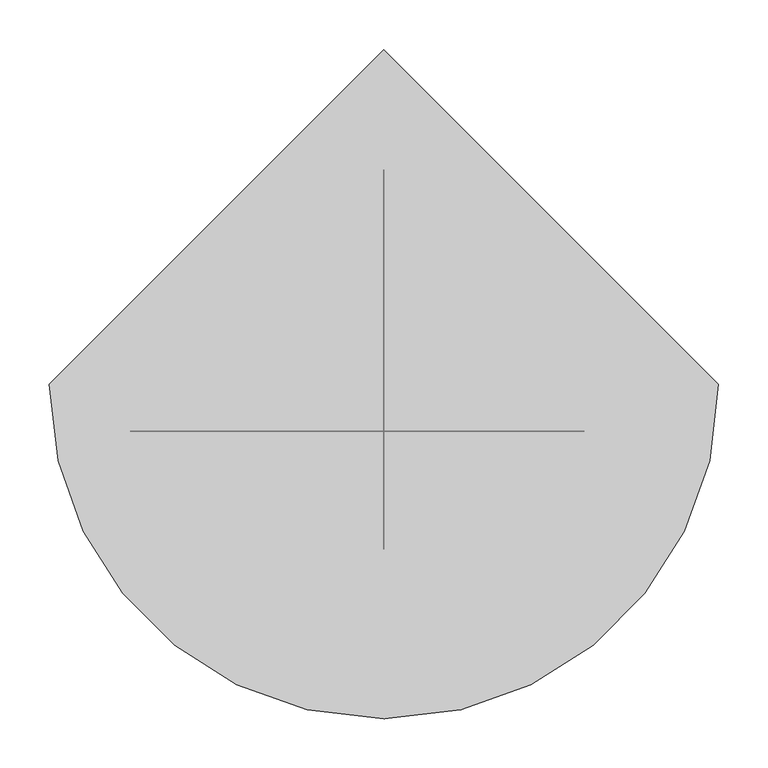
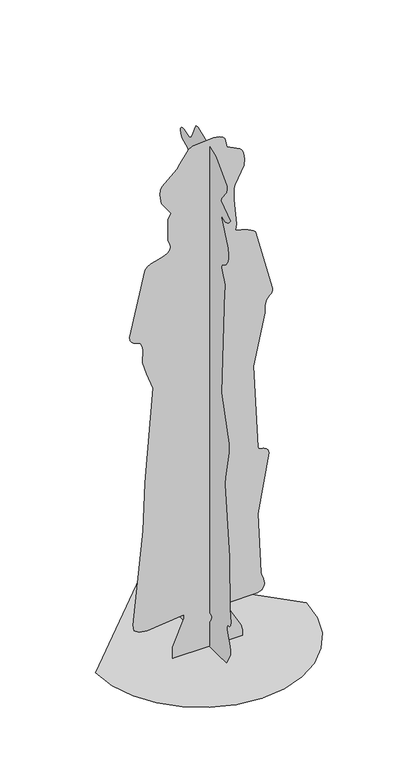
"""IFC4 building model written with IfcOpenShell, lengths in millimetres: proxy geometry, tina 23824 : tina 23824."""

from ifc_helpers import new_model, si_unit, origin, place, context, project, spatial, triangles, source, transform, mapped, element, save


def entourage_2895b76d(model_context):
    return source(origin(), model_context, "Body", "Tessellation", [
        triangles([(-118.6024808, -47.6347378, 38.0857045), (-82.4820657, -47.6347378, 123.5964438), (-82.4078333, -47.6347378, 135.8076171), (-201.8741786, -47.6347378, 123.6873721), (-226.8996859, -47.6347378, 127.3924875), (-242.8002052, -47.6347378, 138.1060324), (-245.9828961, -47.6347378, 157.9872498), (-214.4620912, -47.6347378, 467.6612801), (-208.2590723, -47.6347378, 628.7997002), (-182.2156765, -47.6347378, 942.5936279), (-202.381742, -47.6347378, 998.3094131), (-215.4855752, -47.6347378, 1039.6297834), (-215.821474, -47.6347378, 1048.3149364), (-215.4215529, -47.6347378, 1056.8906485), (-214.7395452, -47.6347378, 1065.4273367), (-214.2301286, -47.6347378, 1073.9983252), (-214.3442568, -47.6347378, 1082.6741764), (-215.5356812, -47.6347378, 1091.525453), (-218.2581349, -47.6347378, 1100.6244616), (-222.7723761, -47.6347378, 1107.0752306), (-229.4309994, -47.6347378, 1111.2517199), (-237.153911, -47.6347378, 1114.3369967), (-244.8601449, -47.6347378, 1117.5141283), (-251.4686441, -47.6347378, 1121.9680716), (-255.900314, -47.6347378, 1128.8818211), (-257.0722446, -47.6347378, 1139.4385895), (-207.1678598, -47.6347378, 1352.9180008), (-199.4588645, -47.6347378, 1360.8821949), (-187.4852313, -47.6347378, 1366.7168678), (-173.049866, -47.6347378, 1371.2959488), (-157.9566194, -47.6347378, 1375.4901695), (-144.0093421, -47.6347378, 1380.175058), (-133.0118575, -47.6347378, 1386.2222179), (-126.7670806, -47.6347378, 1394.5047066), (-125.4318332, -47.6347378, 1401.2801651), (-127.4128987, -47.6347378, 1413.4282608), (-129.6649143, -47.6347378, 1418.6895676), (-132.0486895, -47.6347378, 1423.3336155), (-134.0325437, -47.6347378, 1427.3050301), (-132.6945168, -47.6347378, 1497.2715443), (-129.1053917, -47.6347378, 1508.7544189), (-123.9945118, -47.6347378, 1516.4930454), (-154.1540899, -47.6347378, 1559.4808285), (-159.7585988, -47.6347378, 1590.521957), (-157.2634749, -47.6347378, 1607.9849899), (-153.0368979, -47.6347378, 1617.2900906), (-104.5874569, -47.6347378, 1660.6611351), (-95.4448464, -47.6347378, 1675.8824444), (-68.2647649, -47.6347378, 1712.8963188), (-54.7860727, -47.6347378, 1720.8057198), (13.793251, -47.6347378, 1725.7013512), (32.0821851, -47.6347378, 1722.1345631), (43.5352696, -47.6347378, 1716.6933254), (49.9127328, -47.6347378, 1709.5716671), (56.2159682, -47.6347378, 1680.0680901), (98.2526783, -47.6347378, 1658.6643093), (104.3554853, -47.6347378, 1651.6019497), (108.8919907, -47.6347378, 1641.2540348), (113.2271458, -47.6347378, 1617.3336926), (111.7879713, -47.6347378, 1597.1945148), (82.8123962, -47.6347378, 1541.3868748), (78.3955873, -47.6347378, 1530.355862), (78.221143, -47.6347378, 1494.4090736), (81.1505245, -47.6347378, 1473.5952278), (87.0705392, -47.6347378, 1407.3950535), (83.9407248, -47.6347378, 1386.1879177), (93.3691283, -47.6347378, 1383.7559441), (103.6669826, -47.6347378, 1380.9944847), (114.2487677, -47.6347378, 1377.7940987), (124.5280548, -47.6347378, 1374.0491238), (133.9211951, -47.6347378, 1369.6499737), (141.84176, -47.6347378, 1364.4908409), (147.707027, -47.6347378, 1358.4631565), (203.1565494, -47.6347378, 1147.7562504), (202.6489859, -47.6347378, 1140.2068565), (200.5667729, -47.6347378, 1134.3935486), (197.3998514, -47.6347378, 1129.8329258), (193.6427769, -47.6347378, 1126.0442762), (189.7864171, -47.6347378, 1122.5442719), (186.3244191, -47.6347378, 1118.8530727), (183.7485589, -47.6347378, 1114.4863335), (180.7412388, -47.6347378, 1104.3026527), (179.3224846, -47.6347378, 1093.7014103), (178.983788, -47.6347378, 1082.7502619), (179.2129891, -47.6347378, 1071.5217321), (142.1618895, -47.6347378, 903.7795), (156.0237977, -47.6347378, 623.7611996), (158.5087296, -47.6347378, 617.7901251), (163.2567864, -47.6347378, 614.8626148), (169.444036, -47.6347378, 613.3956259), (176.2446201, -47.6347378, 611.8079321), (182.8317907, -47.6347378, 608.5166722), (188.3815792, -47.6347378, 601.9378587), (192.0662743, -47.6347378, 590.4912827), (156.0237977, -47.6347378, 396.418899), (165.8020344, -47.6347378, 192.9106632), (168.1922955, -47.6347378, 185.5199261), (170.9797162, -47.6347378, 177.5863805), (173.6307353, -47.6347378, 169.2955712), (175.6127183, -47.6347378, 160.8312623), (176.3903053, -47.6347378, 152.379934), (175.4317882, -47.6347378, 144.1253234), (168.3491173, -47.6347378, 133.8915095), (154.6421597, -47.6347378, 127.7701444), (58.9885369, -47.6347378, 127.4899107), (56.2159682, -47.6347378, 116.4005713), (101.0707112, -47.6347378, 37.0993457), (106.6641016, -47.6347378, 18.0541737), (105.8020812, -47.6347378, 0.0), (-118.3148258, -47.6347378, 0.0), (0.0, -54.5513123, 115.1627471), (0.0, -59.6705447, 112.2277973), (0.0, -61.6061461, 107.3080667), (0.0, -59.5796073, 99.6946324), (0.0, -52.8142817, 88.6758101), (0.0, -44.5346181, 79.7484662), (0.0, -38.0847779, 77.4212917), (0.0, -33.3088703, 80.3915047), (0.0, -30.0537933, 87.3554056), (0.0, -27.8620893, 119.17314), (0.0, -145.2091144, 6.8673968), (0.0, -161.5494597, 35.0431167), (0.0, -163.7123909, 41.543994), (0.0, -165.0513535, 56.4646448), (0.0, -162.6425252, 70.0333433), (0.0, -147.9891046, 107.0380432), (0.0, -145.6442986, 119.6101773), (0.0, -147.0779048, 133.0350483), (0.0, -159.447753, 133.9267635), (0.0, -165.7983101, 141.1708889), (0.0, -167.6643299, 152.8364559), (0.0, -161.6821551, 195.066182), (0.0, -158.8307121, 370.4998052), (0.0, -134.8528152, 604.4088561), (0.0, -137.4657826, 630.1117567), (0.0, -156.469192, 724.2417669), (0.0, -156.1305136, 755.5583874), (0.0, -114.2079362, 903.3962385), (0.0, -130.4434278, 1258.6544231), (0.0, -135.0133342, 1270.3422272), (0.0, -134.2635979, 1282.5153214), (0.0, -115.83826, 1329.7483395), (0.0, -116.8218301, 1339.6090748), (0.0, -129.4932496, 1346.1220493), (0.0, -140.4582598, 1355.1042046), (0.0, -148.9049463, 1366.6277744), (0.0, -154.0176883, 1380.767173), (0.0, -154.9836359, 1397.5927448), (0.0, -150.9899389, 1417.1778866), (0.0, -111.0354464, 1505.4037514), (0.0, -130.1557727, 1498.7358444), (0.0, -138.0614948, 1498.201284), (0.0, -145.1534401, 1499.6340454), (0.0, -151.6478203, 1503.109996), (0.0, -157.7617548, 1508.7042767), (0.0, -163.7123909, 1516.4930454), (0.0, -111.0354464, 1555.307246), (0.0, -115.3928657, 1565.6672241), (0.0, -142.5367576, 1601.7699623), (0.0, -145.4540849, 1612.318301), (0.0, -144.305336, 1624.6185677), (0.0, -83.3116117, 1688.3858963), (0.0, 16.4971557, 1727.1999516), (0.0, 26.1092848, 1726.2803856), (0.0, 33.1455581, 1716.0308659), (0.0, 45.9051286, 1684.0145061), (0.0, 54.8352521, 1670.4856808), (0.0, 67.6013152, 1664.1007507), (0.0, 95.5905225, 1672.8907665), (0.0, 103.6679091, 1673.2759174), (0.0, 109.6602941, 1670.5970112), (0.0, 113.1909561, 1665.3155022), (0.0, 113.8794588, 1657.8950249), (0.0, 111.3472188, 1648.7960163), (0.0, 105.2165701, 1638.4815296), (0.0, 102.2760519, 1635.7719566), (0.0, 74.7192446, 1624.6185677), (0.0, 65.7640681, 1614.5842964), (0.0, 62.4319768, 1602.0937798), (0.0, 63.3793663, 1588.1734085), (0.0, 83.0360199, 1538.6726509), (0.0, 77.4992394, 1529.7277027), (0.0, 75.4829062, 1476.4142418), (0.0, 71.8251217, 1469.4614685), (0.0, 16.4971557, 1466.5886787), (0.0, 16.4971557, 1366.7799454), (0.0, 18.8484578, 1360.1880512), (0.0, 52.539621, 1327.9657448), (0.0, 105.3622552, 1231.39911), (0.0, 120.552925, 982.93041), (0.0, 166.2103126, 823.3777943), (0.0, 167.4165798, 801.2900436), (0.0, 164.7089689, 783.190349), (0.0, 144.2060507, 730.9643944), (0.0, 144.0306798, 718.0239052), (0.0, 171.7554501, 645.9398603), (0.0, 186.7994991, 525.8657578), (0.0, 217.1038267, 449.5254684), (0.0, 217.3831338, 436.7788628), (0.0, 207.796982, 424.1436602), (0.0, 134.1002812, 404.8247449), (0.0, 105.2156435, 404.7365962), (0.0, 152.8058437, 209.5887513), (0.0, 152.0635198, 186.4487575), (0.0, 141.0131496, 169.2779487), (0.0, 115.8067122, 150.5668179), (0.0, 57.3786288, 128.2990456), (0.0, 49.7670522, 127.4899107), (0.0, 46.9944834, 116.4005713), (0.0, 56.6344519, 98.9615921), (0.0, 86.162119, 72.0468878), (0.0, 157.830428, 32.1499203), (0.0, 159.4356897, 29.2929136), (0.0, 159.4867404, 24.5244297), (0.0, 158.6367741, 18.6443187), (0.0, 157.534425, 12.4515065), (0.0, 156.8329416, 6.7467698), (0.0, 157.1827568, 2.3299599), (0.0, 159.2361925, 0.0), (0.0, -142.9329725, 0.0), (-339.3492356, 0.0, 0.0), (-330.3783079, -77.756264, 0.0), (-304.8276146, -149.1629065, 0.0), (-264.7450685, -212.1748216, 0.0), (-212.1748216, -264.7450685, 0.0), (-149.1629065, -304.8276146, 0.0), (-77.756264, -330.3783079, 0.0), (0.0, -339.3492356, 0.0), (77.756264, -330.3783079, 0.0), (149.1629065, -304.8276146, 0.0), (212.1748216, -264.7450685, 0.0), (264.7450685, -212.1748216, 0.0), (304.8276146, -149.1629065, 0.0), (330.3783079, -77.756264, 0.0), (339.3492356, 0.0, 0.0), (0.0, 339.3492356, 0.0)], [[108, 109, 110], [107, 108, 110], [107, 110, 1], [106, 107, 1], [106, 1, 2], [106, 2, 3], [105, 106, 3], [5, 6, 7], [4, 5, 7], [4, 7, 8], [3, 4, 8], [105, 3, 8], [104, 105, 8], [103, 104, 8], [102, 103, 8], [101, 102, 8], [100, 101, 8], [99, 100, 8], [98, 99, 8], [97, 98, 8], [96, 97, 8], [95, 96, 8], [95, 8, 9], [94, 95, 9], [93, 94, 9], [92, 93, 9], [91, 92, 9], [90, 91, 9], [89, 90, 9], [88, 89, 9], [87, 88, 9], [86, 87, 9], [86, 9, 10], [86, 10, 11], [85, 86, 11], [84, 85, 11], [84, 11, 12], [84, 12, 13], [84, 13, 14], [84, 14, 15], [84, 15, 16], [84, 16, 17], [83, 84, 17], [83, 17, 18], [82, 83, 18], [82, 18, 19], [81, 82, 19], [80, 81, 19], [80, 19, 20], [79, 80, 20], [78, 79, 20], [77, 78, 20], [76, 77, 20], [75, 76, 20], [74, 75, 20], [73, 74, 20], [72, 73, 20], [71, 72, 20], [70, 71, 20], [69, 70, 20], [68, 69, 20], [67, 68, 20], [66, 67, 20], [66, 20, 21], [66, 21, 22], [66, 22, 23], [66, 23, 24], [66, 24, 25], [66, 25, 26], [66, 26, 27], [66, 27, 28], [66, 28, 29], [66, 29, 30], [66, 30, 31], [66, 31, 32], [66, 32, 33], [66, 33, 34], [66, 34, 35], [65, 66, 35], [64, 65, 35], [64, 35, 36], [64, 36, 37], [63, 64, 37], [63, 37, 38], [63, 38, 39], [63, 39, 40], [63, 40, 41], [63, 41, 42], [62, 63, 42], [61, 62, 42], [61, 42, 43], [61, 43, 44], [61, 44, 45], [61, 45, 46], [61, 46, 47], [61, 47, 48], [60, 61, 48], [59, 60, 48], [58, 59, 48], [57, 58, 48], [56, 57, 48], [55, 56, 48], [55, 48, 49], [55, 49, 50], [55, 50, 51], [55, 51, 52], [55, 52, 53], [55, 53, 54], [218, 219, 220], [115, 123, 124], [115, 124, 125], [114, 115, 125], [114, 125, 126], [113, 114, 126], [113, 126, 127], [217, 218, 220], [155, 156, 157], [122, 123, 115], [122, 115, 116], [121, 122, 116], [216, 217, 220], [215, 216, 220], [214, 215, 220], [213, 214, 220], [212, 213, 220], [211, 212, 220], [210, 211, 220], [210, 220, 121], [209, 210, 121], [112, 113, 127], [112, 127, 128], [183, 184, 185], [180, 181, 182], [121, 116, 117], [209, 121, 117], [209, 117, 118], [209, 118, 119], [209, 119, 120], [208, 209, 120], [154, 155, 157], [153, 154, 157], [152, 153, 157], [151, 152, 157], [150, 151, 157], [163, 164, 165], [162, 163, 165], [162, 165, 166], [128, 129, 130], [128, 130, 131], [112, 128, 131], [112, 131, 132], [111, 112, 132], [120, 111, 132], [208, 120, 132], [208, 132, 133], [207, 208, 133], [206, 207, 133], [205, 206, 133], [204, 205, 133], [203, 204, 133], [202, 203, 133], [202, 133, 134], [182, 183, 185], [202, 134, 135], [180, 182, 185], [162, 166, 167], [161, 162, 167], [160, 161, 167], [159, 160, 167], [158, 159, 167], [157, 158, 167], [157, 167, 168], [150, 157, 168], [201, 202, 135], [200, 201, 135], [199, 200, 135], [198, 199, 135], [197, 198, 135], [196, 197, 135], [195, 196, 135], [195, 135, 136], [194, 195, 136], [194, 136, 137], [193, 194, 137], [192, 193, 137], [191, 192, 137], [191, 137, 138], [190, 191, 138], [190, 138, 139], [189, 190, 139], [188, 189, 139], [188, 139, 140], [188, 140, 141], [188, 141, 142], [187, 188, 142], [187, 142, 143], [186, 187, 143], [185, 186, 143], [185, 143, 144], [185, 144, 145], [185, 145, 146], [185, 146, 147], [185, 147, 148], [185, 148, 149], [185, 149, 150], [185, 150, 168], [170, 171, 172], [170, 172, 173], [169, 170, 173], [169, 173, 174], [169, 174, 175], [169, 175, 176], [168, 169, 176], [168, 176, 177], [168, 177, 178], [185, 168, 178], [185, 178, 179], [180, 185, 179], [235, 236, 221], [234, 235, 221], [234, 221, 222], [233, 234, 222], [233, 222, 223], [233, 223, 224], [232, 233, 224], [231, 232, 224], [231, 224, 225], [231, 225, 226], [231, 226, 227], [231, 227, 228], [231, 228, 229], [231, 229, 230]], closed=False),
    ])


if __name__ == "__main__":
    model = new_model("IFC4")
    model_context = context("Model", 3, world=origin())
    ifc_project = project(units=[si_unit("LENGTHUNIT", "METRE", prefix="MILLI")], contexts=[model_context])
    site = spatial("IfcSite", under=ifc_project)
    building = spatial("IfcBuilding", under=site)
    placement = place(None, origin())
    entourage_shape = entourage_2895b76d(model_context)
    element("IfcBuildingElementProxy", 1, Name="tina 23824 : tina 23824", ObjectType="tina 23824 : tina 23824", at=placement, inside=building, context=model_context, shape_type="MappedRepresentation", body=[
        mapped(entourage_shape, transform((0.0, 0.0, 0.0), x_axis=(1.0, 0.0, 0.0), y_axis=(0.0, 1.0, 0.0), z_axis=(0.0, 0.0, 1.0))),
    ])
    save(model, "model.ifc")

# Revit data of these elements
# Type "tina 23824 : tina 23824"
#   built-in parameter 1005195 = "RPC-8-E23G-6DS7-USQ4-G"
#   Height = 0
